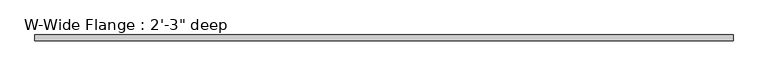
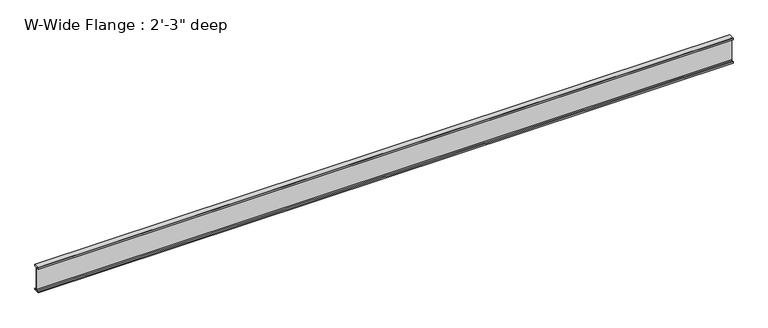
"""IFC4 building model written with IfcOpenShell, lengths in millimetres: beam geometry."""

from ifc_helpers import new_model, si_unit, point, frame, frame_2d, origin, place, context, project, spatial, polyline, circle_curve, trimmed, segment, composite_curve, outline, extrude, source, transform, mapped, element, save


def beam_2afcd037(model_context):
    return source(origin(), model_context, "Body", "SweptSolid", [
        extrude(outline(composite_curve([segment(polyline([(76.2, -308.356), (76.2, -342.9), (-76.2, -342.9), (-76.2, -308.356), (-32.131, -308.356)]), True, "CONTINUOUS"), segment(trimmed(circle_curve(frame_2d((-32.131, -285.75)), 22.606), [point((-32.131, -308.356))], [point((-9.525, -285.75))], True, "CARTESIAN"), True, "CONTINUOUS"), segment(polyline([(-9.525, -285.75), (-9.525, 285.75)]), True, "CONTINUOUS"), segment(trimmed(circle_curve(frame_2d((-32.131, 285.75)), 22.606), [point((-9.525, 285.75))], [point((-32.131, 308.356))], True, "CARTESIAN"), True, "CONTINUOUS"), segment(polyline([(-32.131, 308.356), (-76.2, 308.356), (-76.2, 342.9), (76.2, 342.9), (76.2, 308.356), (32.131, 308.356)]), True, "CONTINUOUS"), segment(trimmed(circle_curve(frame_2d((32.131, 285.75)), 22.606), [point((32.131, 308.356))], [point((9.525, 285.75))], True, "CARTESIAN"), True, "CONTINUOUS"), segment(polyline([(9.525, 285.75), (9.525, -285.75)]), True, "CONTINUOUS"), segment(trimmed(circle_curve(frame_2d((32.131, -285.75)), 22.606), [point((9.525, -285.75))], [point((32.131, -308.356))], True, "CARTESIAN"), True, "CONTINUOUS"), segment(polyline([(32.131, -308.356), (76.2, -308.356)]), True, "CONTINUOUS")], self_intersect=False)), frame((-6974.4000299, 0.0, 0.0), z_axis=(1.0, 0.0, 0.0), x_axis=(0.0, 1.0, 0.0)), (0.0, 0.0, 1.0), 18097.4864736),
    ])


if __name__ == "__main__":
    model = new_model("IFC4")
    model_context = context("Model", 3, world=origin())
    ifc_project = project(units=[si_unit("LENGTHUNIT", "METRE", prefix="MILLI")], contexts=[model_context])
    site = spatial("IfcSite", under=ifc_project)
    building = spatial("IfcBuilding", under=site)
    placement = place(None, origin())
    beam_shape = beam_2afcd037(model_context)
    element("IfcBeam", 1, ObjectType="W-Wide Flange : 2'-3\" deep", at=placement, inside=building, context=model_context, shape_type="MappedRepresentation", body=[
        mapped(beam_shape, transform((0.0, 0.0, 0.0), x_axis=(1.0, 0.0, 0.0), y_axis=(0.0, 1.0, 0.0), z_axis=(0.0, 0.0, 1.0))),
    ])
    save(model, "model.ifc")

# Revit data of these elements
# Type "W-Wide Flange : 2'-3\" deep"
#   Assembly Code = "B10"
#   W = 166
#   Length [instance default] = 5' - 0"
#   bf = 0' - 6"
#   d = 2' - 3"
#   k = 0' - 2 1/4"
#   k2 = 0' - 0.89"
#   tf = 0' - 1.36"
#   tw = 0' - 0 3/4"
#   A = 0.338889 SF
#   Structural Material [instance default] = Steel ASTM A992
# Element 1 (IfcBeam, "W-Wide Flange : 2'-3\" deep")
#   Structural Material = STRUCTURAL STEEL - SEE STRUCT. DWGS
#   Materials on its faces: "STRUCTURAL STEEL - SEE STRUCT. DWGS"
# Materials
#   "Steel ASTM A992": class "Metal", colour RGB 199 199 199, transparency 0, Description = "Structural steel 50ksi", Cost = 0
#   "STRUCTURAL STEEL - SEE STRUCT. DWGS": class "Metal", colour RGB 137 146 153, transparency 0, Description = "Steel, mill finish", Cost = 0
